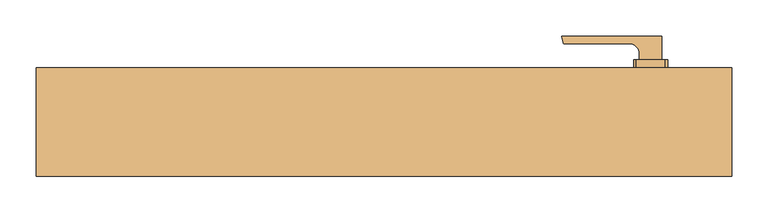
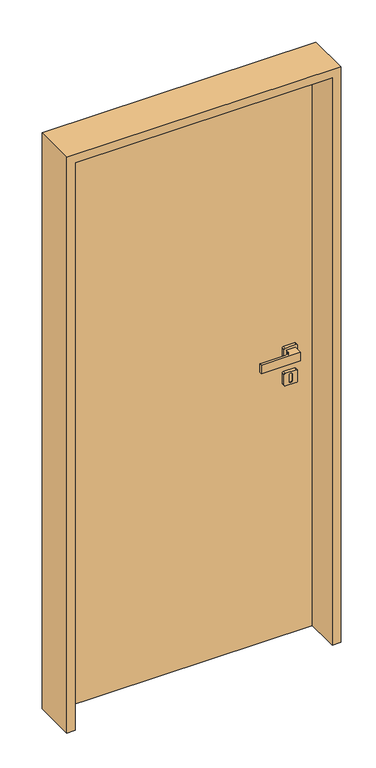
"""IFC4 building model written with IfcOpenShell, lengths in millimetres: door geometry, porta multiplas_growarq : porta giro simples 90 cm_growarq."""

import ifcopenshell
import ifcopenshell.guid

model = None  # the IFC model being written
_history = None  # IfcOwnerHistory: only IFC2X3 demands one
_inside = {}  # id of a spatial element -> (the spatial element, [elements in it])
_under = {}  # id of a project, library or spatial element -> (it, [spatial elements below it])
_declared = {}  # id of a project -> (the project, [libraries it declares])
_typed = {}  # id of a type object -> (the type object, [elements of that type])
_made_of = {}  # id of a material, layer set ... -> (it, [elements and type objects made of it])


def new_model(schema):
    """Start an empty IFC model of exactly this schema.

    Asked for "IFC4X3", IfcOpenShell would pick the latest addendum, in which some entities
    have other attributes; the version numbers below select the first issue.
    IFC2X3 requires an IfcOwnerHistory on every rooted entity: one is made here for all.
    """
    global model, _history
    if schema == "IFC4X3":
        model = ifcopenshell.file(schema_version=(4, 3, 0, 0))
    else:
        model = ifcopenshell.file(schema=schema)
    _inside.clear()
    _under.clear()
    _declared.clear()
    _typed.clear()
    _made_of.clear()
    _history = None
    if model.schema == "IFC2X3":
        org = make("IfcOrganization", Name="unknown")
        user = make(
            "IfcPersonAndOrganization",
            ThePerson=make("IfcPerson", FamilyName="unknown"),
            TheOrganization=org,
        )
        app = make(
            "IfcApplication",
            ApplicationDeveloper=org,
            Version="unknown",
            ApplicationFullName="unknown",
            ApplicationIdentifier="unknown",
        )
        _history = make(
            "IfcOwnerHistory",
            OwningUser=user,
            OwningApplication=app,
            ChangeAction="ADDED",
            CreationDate=0,
        )
    return model


def make(cls, **values):
    """One entity of the class cls with the attributes given. An attribute that is None is left unset."""
    return model.create_entity(
        cls, **{name: value for name, value in values.items() if value is not None}
    )


def rooted(cls, **values):
    """An entity with a GlobalId (a new one), such as an element, a storey or a relation."""
    return make(cls, GlobalId=ifcopenshell.guid.new(), OwnerHistory=_history, **values)


def si_unit(unit_type, name, prefix=None):
    """IfcSIUnit, for example si_unit("LENGTHUNIT", "METRE", prefix="MILLI")."""
    return make("IfcSIUnit", UnitType=unit_type, Prefix=prefix, Name=name)


def assignment(units):
    """IfcUnitAssignment: the units of a project."""
    return None if units is None else make("IfcUnitAssignment", Units=units)


def point(xyz):
    """IfcCartesianPoint."""
    return None if xyz is None else make("IfcCartesianPoint", Coordinates=xyz)


def direction(xyz):
    """IfcDirection."""
    return None if xyz is None else make("IfcDirection", DirectionRatios=xyz)


def frame(location, z_axis=None, x_axis=None):
    """IfcAxis2Placement3D, a coordinate frame: its origin and axes. An axis left out is left unset."""
    return make(
        "IfcAxis2Placement3D",
        Location=point(location),
        Axis=direction(z_axis),
        RefDirection=direction(x_axis),
    )


def frame_2d(location, x_axis=None):
    """IfcAxis2Placement2D, a coordinate frame in the plane: its origin and x axis."""
    return make(
        "IfcAxis2Placement2D", Location=point(location), RefDirection=direction(x_axis)
    )


def origin():
    """The frame at (0, 0, 0) with its axes left unset."""
    return frame((0.0, 0.0, 0.0))


def origin_with_axes():
    """The frame at (0, 0, 0) with the z axis (0, 0, 1) and the x axis (1, 0, 0) written out."""
    return frame((0.0, 0.0, 0.0), z_axis=(0.0, 0.0, 1.0), x_axis=(1.0, 0.0, 0.0))


def place(relative_to, where):
    """IfcLocalPlacement: puts the frame where relative to a parent placement (None: the world)."""
    return make(
        "IfcLocalPlacement", PlacementRelTo=relative_to, RelativePlacement=where
    )


def context(
    kind, dimensions, precision=None, world=None, true_north=None, identifier=None
):
    """IfcGeometricRepresentationContext, for example the 3D "Model" context."""
    return make(
        "IfcGeometricRepresentationContext",
        ContextIdentifier=identifier,
        ContextType=kind,
        CoordinateSpaceDimension=dimensions,
        Precision=precision,
        WorldCoordinateSystem=world,
        TrueNorth=true_north,
    )


def project(units=None, contexts=None):
    """IfcProject with its units and contexts."""
    return rooted(
        "IfcProject",
        Name="project",
        RepresentationContexts=contexts,
        UnitsInContext=assignment(units),
    )


def spatial(cls, under=None, at=None, **own):
    """A site, building, storey or space (cls), placed at a placement, below another one or the project."""
    s = rooted(cls, ObjectPlacement=at, **own)
    if under is not None:
        _under.setdefault(under.id(), (under, []))[1].append(s)
    return s


def polyline(points):
    """IfcPolyline through the points."""
    return make("IfcPolyline", Points=[point(p) for p in points])


def circle_curve(where, radius):
    """IfcCircle in the frame where."""
    return make("IfcCircle", Position=where, Radius=radius)


def trimmed(basis, trim1, trim2, sense, master):
    """IfcTrimmedCurve: the piece of a basis curve between two trims."""
    return make(
        "IfcTrimmedCurve",
        BasisCurve=basis,
        Trim1=trim1,
        Trim2=trim2,
        SenseAgreement=sense,
        MasterRepresentation=master,
    )


def segment(curve, same_sense, transition):
    """IfcCompositeCurveSegment."""
    return make(
        "IfcCompositeCurveSegment",
        Transition=transition,
        SameSense=same_sense,
        ParentCurve=curve,
    )


def composite_curve(segments, self_intersect=None):
    """IfcCompositeCurve: segments joined end to end."""
    return make("IfcCompositeCurve", Segments=segments, SelfIntersect=self_intersect)


def outline(outer, holes=None, kind="AREA"):
    """IfcArbitraryClosedProfileDef: a profile drawn as a closed curve; with holes, ...WithVoids."""
    if holes is None:
        return make("IfcArbitraryClosedProfileDef", ProfileType=kind, OuterCurve=outer)
    return make(
        "IfcArbitraryProfileDefWithVoids",
        ProfileType=kind,
        OuterCurve=outer,
        InnerCurves=holes,
    )


def extrude(swept, where, along, depth):
    """IfcExtrudedAreaSolid: the profile swept, set in the frame where, extruded along a direction by depth."""
    return make(
        "IfcExtrudedAreaSolid",
        SweptArea=swept,
        Position=where,
        ExtrudedDirection=direction(along),
        Depth=depth,
    )


def shape(context_of_items, identifier, shape_type, items):
    """IfcShapeRepresentation: the items that make up one representation, for example the "Body"."""
    return make(
        "IfcShapeRepresentation",
        ContextOfItems=context_of_items,
        RepresentationIdentifier=identifier,
        RepresentationType=shape_type,
        Items=items,
    )


def source(mapping_origin, context_of_items, identifier, shape_type, items):
    """IfcRepresentationMap: a shape defined once, which mapped items show again and again."""
    return make(
        "IfcRepresentationMap",
        MappingOrigin=mapping_origin,
        MappedRepresentation=shape(context_of_items, identifier, shape_type, items),
    )


def transform(
    local_origin,
    x_axis=None,
    y_axis=None,
    z_axis=None,
    scale=None,
    scale2=None,
    scale3=None,
    uniform=True,
):
    """IfcCartesianTransformationOperator3D, or its non-uniform kind. x_axis, y_axis, z_axis: its Axis1, 2, 3."""
    if uniform:
        return make(
            "IfcCartesianTransformationOperator3D",
            Axis1=direction(x_axis),
            Axis2=direction(y_axis),
            LocalOrigin=point(local_origin),
            Scale=scale,
            Axis3=direction(z_axis),
        )
    return make(
        "IfcCartesianTransformationOperator3DnonUniform",
        Axis1=direction(x_axis),
        Axis2=direction(y_axis),
        LocalOrigin=point(local_origin),
        Scale=scale,
        Axis3=direction(z_axis),
        Scale2=scale2,
        Scale3=scale3,
    )


def mapped(mapping_source, mapping_target):
    """IfcMappedItem: shows the shape of a source again, moved by a transform."""
    return make(
        "IfcMappedItem", MappingSource=mapping_source, MappingTarget=mapping_target
    )


def made_of(thing, what):
    """Note that an element or type object is made of a material, layer set ...; save() writes the relation."""
    if what is not None:
        _made_of.setdefault(what.id(), (what, []))[1].append(thing)
    return thing


def element(
    cls,
    number,
    at=None,
    inside=None,
    cuts=None,
    type_object=None,
    material=None,
    context=None,
    identifier="Body",
    shape_type=None,
    held_by="IfcProductDefinitionShape",
    body=None,
    shapes=None,
    **own,
):
    """One element of the class cls, such as IfcWall. Its Tag is "e" and its number.

    at: its placement. inside: the storey or other place that contains it. cuts: it is an
    opening in that element (IfcRelVoidsElement). A single representation is given by context,
    identifier, shape_type and body (its items); several are given by shapes. held_by: the class
    of the entity that holds the representations. save() writes the other relations.
    """
    e = rooted(cls, Tag="e%d" % number, ObjectPlacement=at, **own)
    if body is not None:
        shapes = [shape(context, identifier, shape_type, body)]
    if shapes is not None:
        e.Representation = make(held_by, Representations=shapes)
    if inside is not None:
        _inside.setdefault(inside.id(), (inside, []))[1].append(e)
    if cuts is not None:
        rooted(
            "IfcRelVoidsElement", RelatingBuildingElement=cuts, RelatedOpeningElement=e
        )
    if type_object is not None:
        _typed.setdefault(type_object.id(), (type_object, []))[1].append(e)
    return made_of(e, material)


def aggregate(whole, parts):
    """IfcRelAggregates: a whole, such as a stair, and the parts it consists of."""
    return rooted("IfcRelAggregates", RelatingObject=whole, RelatedObjects=parts)


def save(model, path):
    """Write the relations noted so far, then the file.

    IfcRelAggregates (storeys below a building ...), IfcRelContainedInSpatialStructure (elements
    in a storey), IfcRelDefinesByType, IfcRelAssociatesMaterial and IfcRelDeclares: one each for
    every whole, place, type object, material and project.
    """
    for whole, parts in _under.values():
        aggregate(whole, parts)
    for where, things in _inside.values():
        rooted(
            "IfcRelContainedInSpatialStructure",
            RelatedElements=things,
            RelatingStructure=where,
        )
    for kind, things in _typed.values():
        rooted("IfcRelDefinesByType", RelatedObjects=things, RelatingType=kind)
    for what, things in _made_of.values():
        rooted("IfcRelAssociatesMaterial", RelatedObjects=things, RelatingMaterial=what)
    for by, libraries in _declared.values():
        rooted("IfcRelDeclares", RelatingContext=by, RelatedDefinitions=libraries)
    model.write(path)


def plane_surface(at):
    """IfcPlane: the flat surface through the origin of the frame at, square to its z axis."""
    return make("IfcPlane", Position=at)


def cylinder_surface(at, radius):
    """IfcCylindricalSurface: all points at the distance radius from the z axis of the frame at."""
    return make("IfcCylindricalSurface", Position=at, Radius=radius)


def revolved_surface(curve, axis_point, axis_direction):
    """IfcSurfaceOfRevolution: the curve turned about the line through axis_point along axis_direction."""
    return make(
        "IfcSurfaceOfRevolution",
        SweptCurve=make("IfcArbitraryOpenProfileDef", ProfileType="CURVE", Curve=curve),
        AxisPosition=make("IfcAxis1Placement", Location=point(axis_point), Axis=direction(axis_direction)),
    )


def advanced_brep(points, edges, surfaces, faces):
    """IfcAdvancedBrep: a solid bounded by faces that lie on surfaces and meet in shared edges.

    An edge is (start, end): straight between two places in points (the first is 0);
    or (start, end, curve); or (start, end, curve, False) where it runs against its curve.
    A face is (place in surfaces, loops), or (place, loops, False) where it looks against
    its surface's normal. A loop lists edges by number (the first is 1), with a minus sign
    where the edge is run from its end to its start. The first loop is the outer one.
    """
    corners = [point(p) for p in points]
    vertices = [make("IfcVertexPoint", VertexGeometry=c) for c in corners]
    made = []
    for start, end, *more in edges:
        made.append(
            make(
                "IfcEdgeCurve",
                EdgeStart=vertices[start],
                EdgeEnd=vertices[end],
                EdgeGeometry=more[0] if more else make("IfcPolyline", Points=[corners[start], corners[end]]),
                SameSense=more[1] if len(more) > 1 else True,
            )
        )
    hull = []
    for where, loops, *sense in faces:
        bounds = []
        for j, loop in enumerate(loops):
            ring = [make("IfcOrientedEdge", EdgeElement=made[abs(k) - 1], Orientation=k > 0) for k in loop]
            bounds.append(
                make(
                    "IfcFaceOuterBound" if j == 0 else "IfcFaceBound",
                    Bound=make("IfcEdgeLoop", EdgeList=ring),
                    Orientation=True,
                )
            )
        hull.append(make("IfcAdvancedFace", Bounds=bounds, FaceSurface=surfaces[where], SameSense=sense[0] if sense else True))
    return make("IfcAdvancedBrep", Outer=make("IfcClosedShell", CfsFaces=hull))


def door_3435e1a8(model_context):
    return source(origin(), model_context, "Body", "SolidModel", [
        advanced_brep(
        [(387.5247906, 86.0, 975.2140175), (391.5247906, 86.0, 971.2140175), (391.5247906, 86.0, 932.3348635), (387.5247906, 86.0, 928.3348635), (348.475196, 86.0, 928.3348635), (344.475196, 86.0, 932.3348635), (344.475196, 86.0, 971.2071442), (348.4820692, 86.0, 975.2140175), (373.0036235, 86.0, 963.1453546), (362.9935514, 86.0, 963.1453546), (362.9935514, 86.0, 940.4035264), (373.0036235, 86.0, 940.4035264), (387.5247906, 75.0, 975.2140175), (348.4820692, 75.0, 975.2140175), (344.475196, 75.0, 971.2071442), (344.475196, 75.0, 932.3348635), (348.475196, 75.0, 928.3348635), (387.5247906, 75.0, 928.3348635), (391.5247906, 75.0, 932.3348635), (391.5247906, 75.0, 971.2140175), (373.0036235, 84.0, 940.4035264), (362.9935514, 84.0, 940.4035264), (362.9935514, 84.0, 963.1453546), (373.0036235, 84.0, 963.1453546)],
        [
            (0, 1, circle_curve(frame((387.5247906, 86.0, 971.2140175), z_axis=(0.0, 1.0, 0.0), x_axis=(1.0, 0.0, 0.0)), 4.0)),
            (1, 2),
            (2, 3, circle_curve(frame((387.5247906, 86.0, 932.3348635), z_axis=(0.0, 1.0, 0.0), x_axis=(1.0, 0.0, 0.0)), 4.0)),
            (3, 4),
            (4, 5, circle_curve(frame((348.475196, 86.0, 932.3348635), z_axis=(0.0, 1.0, 0.0), x_axis=(1.0, 0.0, 0.0)), 4.0)),
            (5, 6),
            (6, 7, circle_curve(frame((348.4820692, 86.0, 971.2071442), z_axis=(0.0, 1.0, 0.0), x_axis=(1.0, 0.0, 0.0)), 4.0068732)),
            (7, 0),
            (8, 9, circle_curve(frame((367.9985874, 86.0, 963.1453546), z_axis=(0.0, -1.0, 0.0), x_axis=(1.0, 0.0, 0.0)), 5.0050361)),
            (9, 10),
            (10, 11, circle_curve(frame((367.9985874, 86.0, 940.4035264), z_axis=(0.0, -1.0, 0.0), x_axis=(1.0, 0.0, 0.0)), 5.0050361)),
            (11, 8),
            (12, 13),
            (13, 14, circle_curve(frame((348.4820692, 75.0, 971.2071442), z_axis=(0.0, -1.0, 0.0), x_axis=(1.0, 0.0, 0.0)), 4.0068732)),
            (14, 15),
            (15, 16, circle_curve(frame((348.475196, 75.0, 932.3348635), z_axis=(0.0, -1.0, 0.0), x_axis=(1.0, 0.0, 0.0)), 4.0)),
            (16, 17),
            (17, 18, circle_curve(frame((387.5247906, 75.0, 932.3348635), z_axis=(0.0, -1.0, 0.0), x_axis=(1.0, 0.0, 0.0)), 4.0)),
            (18, 19),
            (19, 12, circle_curve(frame((387.5247906, 75.0, 971.2140175), z_axis=(0.0, -1.0, 0.0), x_axis=(1.0, 0.0, 0.0)), 4.0)),
            (7, 13),
            (12, 0),
            (6, 14),
            (5, 15),
            (4, 16),
            (3, 17),
            (2, 18),
            (1, 19),
            (20, 21, circle_curve(frame((367.9985874, 84.0, 940.4035264), z_axis=(0.0, 1.0, 0.0), x_axis=(1.0, 0.0, 0.0)), 5.0050361)),
            (21, 22),
            (22, 23, circle_curve(frame((367.9985874, 84.0, 963.1453546), z_axis=(0.0, 1.0, 0.0), x_axis=(1.0, 0.0, 0.0)), 5.0050361)),
            (23, 20),
            (23, 8),
            (11, 20),
            (21, 10),
            (9, 22),
        ],
        [
            plane_surface(frame((348.4781039, 86.0, 975.2140175), z_axis=(0.0, 1.0, 0.0), x_axis=(-1.0, 0.0, 0.0))),
            plane_surface(frame((348.4781039, 75.0, 975.2140175), z_axis=(0.0, -1.0, 0.0), x_axis=(1.0, 0.0, 0.0))),
            plane_surface(frame((387.5247906, 86.0, 975.2140175), z_axis=(0.0, 0.0, 1.0), x_axis=(0.0, -1.0, 0.0))),
            cylinder_surface(frame((348.4820692, 75.0, 971.2071442), z_axis=(0.0, 1.0, 0.0), x_axis=(1.0, 0.0, 0.0)), 4.0068732),
            plane_surface(frame((344.475196, 86.0, 971.2071442), z_axis=(-1.0, 0.0, 0.0), x_axis=(0.0, -1.0, 0.0))),
            cylinder_surface(frame((348.475196, 75.0, 932.3348635), z_axis=(0.0, 1.0, 0.0), x_axis=(1.0, 0.0, 0.0)), 4.0),
            plane_surface(frame((348.475196, 86.0, 928.3348635), z_axis=(0.0, 0.0, -1.0), x_axis=(0.0, -1.0, 0.0))),
            cylinder_surface(frame((387.5247906, 75.0, 932.3348635), z_axis=(0.0, 1.0, 0.0), x_axis=(1.0, 0.0, 0.0)), 4.0),
            plane_surface(frame((391.5247906, 86.0, 932.3348635), z_axis=(1.0, 0.0, 0.0), x_axis=(0.0, -1.0, 0.0))),
            cylinder_surface(frame((387.5247906, 75.0, 971.2140175), z_axis=(0.0, 1.0, 0.0), x_axis=(1.0, 0.0, 0.0)), 4.0),
            plane_surface(frame((373.0036235, 84.0, 952.9958878), z_axis=(0.0, 1.0, 0.0), x_axis=(0.0, 0.0, -1.0))),
            plane_surface(frame((373.0036235, 86.0, 940.4035264), z_axis=(-1.0, 0.0, 0.0), x_axis=(0.0, -1.0, 0.0))),
            plane_surface(frame((362.9935514, 86.0, 963.1453546), z_axis=(1.0, 0.0, 0.0), x_axis=(0.0, -1.0, 0.0))),
            revolved_surface(polyline([(373.0036235, 86.0, 940.4035264), (373.0036235, 84.0, 940.4035264)]), (367.9985874, 84.0, 940.4035264), (0.0, 1.0, 0.0)),
            revolved_surface(polyline([(373.0036235, 86.0, 963.1453546), (373.0036235, 84.0, 963.1453546)]), (367.9985874, 84.0, 963.1453546), (0.0, 1.0, 0.0)),
        ],
        [
            (0, [[1, 2, 3, 4, 5, 6, 7, 8], [9, 10, 11, 12]]),
            (1, [[13, 14, 15, 16, 17, 18, 19, 20]]),
            (2, [[21, -13, 22, -8]]),
            (3, [[23, -14, -21, -7]]),
            (4, [[24, -15, -23, -6]]),
            (5, [[25, -16, -24, -5]]),
            (6, [[26, -17, -25, -4]]),
            (7, [[27, -18, -26, -3]]),
            (8, [[28, -19, -27, -2]]),
            (9, [[-22, -20, -28, -1]]),
            (10, [[29, 30, 31, 32]]),
            (11, [[33, -12, 34, -32]]),
            (12, [[35, -10, 36, -30]]),
            (13, [[-34, -11, -35, -29]]),
            (14, [[-36, -9, -33, -31]]),
        ],
    ),
        advanced_brep(
        [(387.5247906, 86.0, 1068.227973), (391.5247906, 86.0, 1064.227973), (391.5247906, 86.0, 1025.3488191), (387.5247906, 86.0, 1021.3488191), (348.475196, 86.0, 1021.3488191), (344.475196, 86.0, 1025.3488191), (344.475196, 86.0, 1064.2210998), (348.4820692, 86.0, 1068.227973), (387.5247906, 75.0, 1068.227973), (348.4820692, 75.0, 1068.227973), (344.475196, 75.0, 1064.2210998), (344.475196, 75.0, 1025.3488191), (348.475196, 75.0, 1021.3488191), (387.5247906, 75.0, 1021.3488191), (391.5247906, 75.0, 1025.3488191), (391.5247906, 75.0, 1064.227973)],
        [
            (0, 1, circle_curve(frame((387.5247906, 86.0, 1064.227973), z_axis=(0.0, 1.0, 0.0), x_axis=(1.0, 0.0, 0.0)), 4.0)),
            (1, 2),
            (2, 3, circle_curve(frame((387.5247906, 86.0, 1025.3488191), z_axis=(0.0, 1.0, 0.0), x_axis=(1.0, 0.0, 0.0)), 4.0)),
            (3, 4),
            (4, 5, circle_curve(frame((348.475196, 86.0, 1025.3488191), z_axis=(0.0, 1.0, 0.0), x_axis=(1.0, 0.0, 0.0)), 4.0)),
            (5, 6),
            (6, 7, circle_curve(frame((348.4820692, 86.0, 1064.2210998), z_axis=(0.0, 1.0, 0.0), x_axis=(1.0, 0.0, 0.0)), 4.0068732)),
            (7, 0),
            (8, 9),
            (9, 10, circle_curve(frame((348.4820692, 75.0, 1064.2210998), z_axis=(0.0, -1.0, 0.0), x_axis=(1.0, 0.0, 0.0)), 4.0068732)),
            (10, 11),
            (11, 12, circle_curve(frame((348.475196, 75.0, 1025.3488191), z_axis=(0.0, -1.0, 0.0), x_axis=(1.0, 0.0, 0.0)), 4.0)),
            (12, 13),
            (13, 14, circle_curve(frame((387.5247906, 75.0, 1025.3488191), z_axis=(0.0, -1.0, 0.0), x_axis=(1.0, 0.0, 0.0)), 4.0)),
            (14, 15),
            (15, 8, circle_curve(frame((387.5247906, 75.0, 1064.227973), z_axis=(0.0, -1.0, 0.0), x_axis=(1.0, 0.0, 0.0)), 4.0)),
            (7, 9),
            (8, 0),
            (6, 10),
            (5, 11),
            (4, 12),
            (3, 13),
            (2, 14),
            (1, 15),
        ],
        [
            plane_surface(frame((348.4781039, 86.0, 975.2140175), z_axis=(0.0, 1.0, 0.0), x_axis=(-1.0, 0.0, 0.0))),
            plane_surface(frame((348.4781039, 75.0, 975.2140175), z_axis=(0.0, -1.0, 0.0), x_axis=(1.0, 0.0, 0.0))),
            plane_surface(frame((387.5247906, 86.0, 1068.227973), z_axis=(0.0, 0.0, 1.0), x_axis=(0.0, -1.0, 0.0))),
            cylinder_surface(frame((348.4820692, 75.0, 1064.2210998), z_axis=(0.0, 1.0, 0.0), x_axis=(1.0, 0.0, 0.0)), 4.0068732),
            plane_surface(frame((344.475196, 86.0, 1064.2210998), z_axis=(-1.0, 0.0, 0.0), x_axis=(0.0, -1.0, 0.0))),
            cylinder_surface(frame((348.475196, 75.0, 1025.3488191), z_axis=(0.0, 1.0, 0.0), x_axis=(1.0, 0.0, 0.0)), 4.0),
            plane_surface(frame((348.475196, 86.0, 1021.3488191), z_axis=(0.0, 0.0, -1.0), x_axis=(0.0, -1.0, 0.0))),
            cylinder_surface(frame((387.5247906, 75.0, 1025.3488191), z_axis=(0.0, 1.0, 0.0), x_axis=(1.0, 0.0, 0.0)), 4.0),
            plane_surface(frame((391.5247906, 86.0, 1025.3488191), z_axis=(1.0, 0.0, 0.0), x_axis=(0.0, -1.0, 0.0))),
            cylinder_surface(frame((387.5247906, 75.0, 1064.227973), z_axis=(0.0, 1.0, 0.0), x_axis=(1.0, 0.0, 0.0)), 4.0),
        ],
        [
            (0, [[1, 2, 3, 4, 5, 6, 7, 8]]),
            (1, [[9, 10, 11, 12, 13, 14, 15, 16]]),
            (2, [[17, -9, 18, -8]]),
            (3, [[19, -10, -17, -7]]),
            (4, [[20, -11, -19, -6]]),
            (5, [[21, -12, -20, -5]]),
            (6, [[22, -13, -21, -4]]),
            (7, [[23, -14, -22, -3]]),
            (8, [[24, -15, -23, -2]]),
            (9, [[-18, -16, -24, -1]]),
        ],
    ),
        extrude(outline(composite_curve([segment(polyline([(383.5247906, 118.5150355), (383.5247906, 86.7793682), (352.475196, 86.7793682), (352.475196, 93.5981558)]), True, "CONTINUOUS"), segment(trimmed(circle_curve(frame_2d((337.4483579, 93.5981558)), 15.0268381), [point((352.475196, 93.5981558))], [point((337.4483579, 108.6249939))], True, "CARTESIAN"), True, "CONTINUOUS"), segment(polyline([(337.4483579, 108.6249939), (248.1590205, 108.6249939)]), True, "CONTINUOUS"), segment(trimmed(circle_curve(frame_2d((248.1590205, 109.6372538)), 1.0122598), [point((248.1590205, 108.6249939))], [point((247.1621392, 109.4614767))], False, "CARTESIAN"), True, "CONTINUOUS"), segment(polyline([(247.1621392, 109.4614767), (245.5657525, 118.5150355), (383.5247906, 118.5150355)]), True, "CONTINUOUS")], self_intersect=False)), frame((0.0, 0.0, 1029.3488191), z_axis=(0.0, 0.0, 1.0), x_axis=(1.0, 0.0, 0.0)), (0.0, 0.0, 1.0), 30.8791539),
        advanced_brep(
        [(387.5247906, 34.0, 975.2140175), (348.4820692, 34.0, 975.2140175), (344.475196, 34.0, 971.2071442), (344.475196, 34.0, 932.3348635), (348.475196, 34.0, 928.3348635), (387.5247906, 34.0, 928.3348635), (391.5247906, 34.0, 932.3348635), (391.5247906, 34.0, 971.2140175), (373.0036235, 34.0, 963.1453546), (373.0036235, 34.0, 940.4035264), (362.9935514, 34.0, 940.4035264), (362.9935514, 34.0, 963.1453546), (387.5247906, 45.0, 975.2140175), (391.5247906, 45.0, 971.2140175), (391.5247906, 45.0, 932.3348635), (387.5247906, 45.0, 928.3348635), (348.475196, 45.0, 928.3348635), (344.475196, 45.0, 932.3348635), (344.475196, 45.0, 971.2071442), (348.4820692, 45.0, 975.2140175), (373.0036235, 36.0, 940.4035264), (373.0036235, 36.0, 963.1453546), (362.9935514, 36.0, 963.1453546), (362.9935514, 36.0, 940.4035264)],
        [
            (0, 1),
            (1, 2, circle_curve(frame((348.4820692, 34.0, 971.2071442), z_axis=(0.0, -1.0, 0.0), x_axis=(1.0, 0.0, 0.0)), 4.0068732)),
            (2, 3),
            (3, 4, circle_curve(frame((348.475196, 34.0, 932.3348635), z_axis=(0.0, -1.0, 0.0), x_axis=(1.0, 0.0, 0.0)), 4.0)),
            (4, 5),
            (5, 6, circle_curve(frame((387.5247906, 34.0, 932.3348635), z_axis=(0.0, -1.0, 0.0), x_axis=(1.0, 0.0, 0.0)), 4.0)),
            (6, 7),
            (7, 0, circle_curve(frame((387.5247906, 34.0, 971.2140175), z_axis=(0.0, -1.0, 0.0), x_axis=(1.0, 0.0, 0.0)), 4.0)),
            (8, 9),
            (9, 10, circle_curve(frame((367.9985874, 34.0, 940.4035264), z_axis=(0.0, 1.0, 0.0), x_axis=(1.0, 0.0, 0.0)), 5.0050361)),
            (10, 11),
            (11, 8, circle_curve(frame((367.9985874, 34.0, 963.1453546), z_axis=(0.0, 1.0, 0.0), x_axis=(1.0, 0.0, 0.0)), 5.0050361)),
            (12, 13, circle_curve(frame((387.5247906, 45.0, 971.2140175), z_axis=(0.0, 1.0, 0.0), x_axis=(1.0, 0.0, 0.0)), 4.0)),
            (13, 14),
            (14, 15, circle_curve(frame((387.5247906, 45.0, 932.3348635), z_axis=(0.0, 1.0, 0.0), x_axis=(1.0, 0.0, 0.0)), 4.0)),
            (15, 16),
            (16, 17, circle_curve(frame((348.475196, 45.0, 932.3348635), z_axis=(0.0, 1.0, 0.0), x_axis=(1.0, 0.0, 0.0)), 4.0)),
            (17, 18),
            (18, 19, circle_curve(frame((348.4820692, 45.0, 971.2071442), z_axis=(0.0, 1.0, 0.0), x_axis=(1.0, 0.0, 0.0)), 4.0068732)),
            (19, 12),
            (0, 12),
            (19, 1),
            (18, 2),
            (17, 3),
            (16, 4),
            (15, 5),
            (14, 6),
            (13, 7),
            (20, 21),
            (21, 22, circle_curve(frame((367.9985874, 36.0, 963.1453546), z_axis=(0.0, -1.0, 0.0), x_axis=(1.0, 0.0, 0.0)), 5.0050361)),
            (22, 23),
            (23, 20, circle_curve(frame((367.9985874, 36.0, 940.4035264), z_axis=(0.0, -1.0, 0.0), x_axis=(1.0, 0.0, 0.0)), 5.0050361)),
            (20, 9),
            (8, 21),
            (22, 11),
            (10, 23),
        ],
        [
            plane_surface(frame((348.4781039, 34.0, 975.2140175), z_axis=(0.0, -1.0, 0.0), x_axis=(-1.0, 0.0, 0.0))),
            plane_surface(frame((348.4781039, 45.0, 975.2140175), z_axis=(0.0, 1.0, 0.0), x_axis=(1.0, 0.0, 0.0))),
            plane_surface(frame((387.5247906, 34.0, 975.2140175), z_axis=(0.0, 0.0, 1.0), x_axis=(0.0, 1.0, 0.0))),
            cylinder_surface(frame((348.4820692, 45.0, 971.2071442), z_axis=(0.0, -1.0, 0.0), x_axis=(1.0, 0.0, 0.0)), 4.0068732),
            plane_surface(frame((344.475196, 34.0, 971.2071442), z_axis=(-1.0, 0.0, 0.0), x_axis=(0.0, 1.0, 0.0))),
            cylinder_surface(frame((348.475196, 45.0, 932.3348635), z_axis=(0.0, -1.0, 0.0), x_axis=(1.0, 0.0, 0.0)), 4.0),
            plane_surface(frame((348.475196, 34.0, 928.3348635), z_axis=(0.0, 0.0, -1.0), x_axis=(0.0, 1.0, 0.0))),
            cylinder_surface(frame((387.5247906, 45.0, 932.3348635), z_axis=(0.0, -1.0, 0.0), x_axis=(1.0, 0.0, 0.0)), 4.0),
            plane_surface(frame((391.5247906, 34.0, 932.3348635), z_axis=(1.0, 0.0, 0.0), x_axis=(0.0, 1.0, 0.0))),
            cylinder_surface(frame((387.5247906, 45.0, 971.2140175), z_axis=(0.0, -1.0, 0.0), x_axis=(1.0, 0.0, 0.0)), 4.0),
            plane_surface(frame((373.0036235, 36.0, 952.9958878), z_axis=(0.0, -1.0, 0.0), x_axis=(0.0, 0.0, -1.0))),
            plane_surface(frame((373.0036235, 34.0, 940.4035264), z_axis=(-1.0, 0.0, 0.0), x_axis=(0.0, 1.0, 0.0))),
            plane_surface(frame((362.9935514, 34.0, 963.1453546), z_axis=(1.0, 0.0, 0.0), x_axis=(0.0, 1.0, 0.0))),
            revolved_surface(polyline([(373.0036235, 34.0, 940.4035264), (373.0036235, 36.0, 940.4035264)]), (367.9985874, 36.0, 940.4035264), (0.0, -1.0, 0.0)),
            revolved_surface(polyline([(373.0036235, 34.0, 963.1453546), (373.0036235, 36.0, 963.1453546)]), (367.9985874, 36.0, 963.1453546), (0.0, -1.0, 0.0)),
        ],
        [
            (0, [[1, 2, 3, 4, 5, 6, 7, 8], [9, 10, 11, 12]]),
            (1, [[13, 14, 15, 16, 17, 18, 19, 20]]),
            (2, [[-1, 21, -20, 22]]),
            (3, [[-2, -22, -19, 23]]),
            (4, [[-3, -23, -18, 24]]),
            (5, [[-4, -24, -17, 25]]),
            (6, [[-5, -25, -16, 26]]),
            (7, [[-6, -26, -15, 27]]),
            (8, [[-7, -27, -14, 28]]),
            (9, [[-8, -28, -13, -21]]),
            (10, [[29, 30, 31, 32]]),
            (11, [[-29, 33, -9, 34]]),
            (12, [[-31, 35, -11, 36]]),
            (13, [[-32, -36, -10, -33]]),
            (14, [[-30, -34, -12, -35]]),
        ],
    ),
        advanced_brep(
        [(387.5247906, 34.0, 1068.227973), (348.4820692, 34.0, 1068.227973), (344.475196, 34.0, 1064.2210998), (344.475196, 34.0, 1025.3488191), (348.475196, 34.0, 1021.3488191), (387.5247906, 34.0, 1021.3488191), (391.5247906, 34.0, 1025.3488191), (391.5247906, 34.0, 1064.227973), (387.5247906, 45.0, 1068.227973), (391.5247906, 45.0, 1064.227973), (391.5247906, 45.0, 1025.3488191), (387.5247906, 45.0, 1021.3488191), (348.475196, 45.0, 1021.3488191), (344.475196, 45.0, 1025.3488191), (344.475196, 45.0, 1064.2210998), (348.4820692, 45.0, 1068.227973)],
        [
            (0, 1),
            (1, 2, circle_curve(frame((348.4820692, 34.0, 1064.2210998), z_axis=(0.0, -1.0, 0.0), x_axis=(1.0, 0.0, 0.0)), 4.0068732)),
            (2, 3),
            (3, 4, circle_curve(frame((348.475196, 34.0, 1025.3488191), z_axis=(0.0, -1.0, 0.0), x_axis=(1.0, 0.0, 0.0)), 4.0)),
            (4, 5),
            (5, 6, circle_curve(frame((387.5247906, 34.0, 1025.3488191), z_axis=(0.0, -1.0, 0.0), x_axis=(1.0, 0.0, 0.0)), 4.0)),
            (6, 7),
            (7, 0, circle_curve(frame((387.5247906, 34.0, 1064.227973), z_axis=(0.0, -1.0, 0.0), x_axis=(1.0, 0.0, 0.0)), 4.0)),
            (8, 9, circle_curve(frame((387.5247906, 45.0, 1064.227973), z_axis=(0.0, 1.0, 0.0), x_axis=(1.0, 0.0, 0.0)), 4.0)),
            (9, 10),
            (10, 11, circle_curve(frame((387.5247906, 45.0, 1025.3488191), z_axis=(0.0, 1.0, 0.0), x_axis=(1.0, 0.0, 0.0)), 4.0)),
            (11, 12),
            (12, 13, circle_curve(frame((348.475196, 45.0, 1025.3488191), z_axis=(0.0, 1.0, 0.0), x_axis=(1.0, 0.0, 0.0)), 4.0)),
            (13, 14),
            (14, 15, circle_curve(frame((348.4820692, 45.0, 1064.2210998), z_axis=(0.0, 1.0, 0.0), x_axis=(1.0, 0.0, 0.0)), 4.0068732)),
            (15, 8),
            (0, 8),
            (15, 1),
            (14, 2),
            (13, 3),
            (12, 4),
            (11, 5),
            (10, 6),
            (9, 7),
        ],
        [
            plane_surface(frame((348.4781039, 34.0, 975.2140175), z_axis=(0.0, -1.0, 0.0), x_axis=(-1.0, 0.0, 0.0))),
            plane_surface(frame((348.4781039, 45.0, 975.2140175), z_axis=(0.0, 1.0, 0.0), x_axis=(1.0, 0.0, 0.0))),
            plane_surface(frame((387.5247906, 34.0, 1068.227973), z_axis=(0.0, 0.0, 1.0), x_axis=(0.0, 1.0, 0.0))),
            cylinder_surface(frame((348.4820692, 45.0, 1064.2210998), z_axis=(0.0, -1.0, 0.0), x_axis=(1.0, 0.0, 0.0)), 4.0068732),
            plane_surface(frame((344.475196, 34.0, 1064.2210998), z_axis=(-1.0, 0.0, 0.0), x_axis=(0.0, 1.0, 0.0))),
            cylinder_surface(frame((348.475196, 45.0, 1025.3488191), z_axis=(0.0, -1.0, 0.0), x_axis=(1.0, 0.0, 0.0)), 4.0),
            plane_surface(frame((348.475196, 34.0, 1021.3488191), z_axis=(0.0, 0.0, -1.0), x_axis=(0.0, 1.0, 0.0))),
            cylinder_surface(frame((387.5247906, 45.0, 1025.3488191), z_axis=(0.0, -1.0, 0.0), x_axis=(1.0, 0.0, 0.0)), 4.0),
            plane_surface(frame((391.5247906, 34.0, 1025.3488191), z_axis=(1.0, 0.0, 0.0), x_axis=(0.0, 1.0, 0.0))),
            cylinder_surface(frame((387.5247906, 45.0, 1064.227973), z_axis=(0.0, -1.0, 0.0), x_axis=(1.0, 0.0, 0.0)), 4.0),
        ],
        [
            (0, [[1, 2, 3, 4, 5, 6, 7, 8]]),
            (1, [[9, 10, 11, 12, 13, 14, 15, 16]]),
            (2, [[-1, 17, -16, 18]]),
            (3, [[-2, -18, -15, 19]]),
            (4, [[-3, -19, -14, 20]]),
            (5, [[-4, -20, -13, 21]]),
            (6, [[-5, -21, -12, 22]]),
            (7, [[-6, -22, -11, 23]]),
            (8, [[-7, -23, -10, 24]]),
            (9, [[-8, -24, -9, -17]]),
        ],
    ),
        extrude(outline(composite_curve([segment(polyline([(383.5247906, 1.4849645), (245.5657525, 1.4849645), (247.1621392, 10.5385233)]), True, "CONTINUOUS"), segment(trimmed(circle_curve(frame_2d((248.1590205, 10.3627462)), 1.0122598), [point((247.1621392, 10.5385233))], [point((248.1590205, 11.3750061))], False, "CARTESIAN"), True, "CONTINUOUS"), segment(polyline([(248.1590205, 11.3750061), (337.4483579, 11.3750061)]), True, "CONTINUOUS"), segment(trimmed(circle_curve(frame_2d((337.4483579, 26.4018442)), 15.0268381), [point((337.4483579, 11.3750061))], [point((352.475196, 26.4018442))], True, "CARTESIAN"), True, "CONTINUOUS"), segment(polyline([(352.475196, 26.4018442), (352.475196, 33.2206318), (383.5247906, 33.2206318), (383.5247906, 1.4849645)]), True, "CONTINUOUS")], self_intersect=False)), frame((0.0, 0.0, 1029.3488191), z_axis=(0.0, 0.0, 1.0), x_axis=(1.0, 0.0, 0.0)), (0.0, 0.0, 1.0), 30.8791539),
        extrude(outline(polyline([(448.0, 45.0), (-448.0, 45.0), (-448.0, 75.0), (448.0, 75.0), (448.0, 45.0)])), origin_with_axes(), (0.0, 0.0, 1.0), 2098.0),
        extrude(outline(polyline([(0.0, 450.0), (0.0, 480.0), (2130.0, 480.0), (2130.0, -480.0), (0.0, -480.0), (0.0, -450.0), (2100.0, -450.0), (2100.0, 450.0), (0.0, 450.0)])), frame((0.0, -75.0, 0.0), z_axis=(0.0, 1.0, 0.0), x_axis=(0.0, 0.0, 1.0)), (0.0, 0.0, 1.0), 150.0),
    ])


if __name__ == "__main__":
    model = new_model("IFC4")
    model_context = context("Model", 3, world=origin())
    ifc_project = project(units=[si_unit("LENGTHUNIT", "METRE", prefix="MILLI")], contexts=[model_context])
    site = spatial("IfcSite", under=ifc_project)
    building = spatial("IfcBuilding", under=site)
    placement = place(None, origin())
    door_shape = door_3435e1a8(model_context)
    element("IfcDoor", 1, ObjectType="porta multiplas_growarq : porta giro simples 90 cm_growarq", at=placement, inside=building, context=model_context, shape_type="MappedRepresentation", body=[
        mapped(door_shape, transform((0.0, 0.0, 0.0), x_axis=(1.0, 0.0, 0.0), y_axis=(0.0, 1.0, 0.0), z_axis=(0.0, 0.0, 1.0))),
    ])
    save(model, "model.ifc")

# Revit data of these elements
# Type "porta multiplas_growarq : porta giro simples 90 cm_growarq"
#   Type Mark = "P01"
#   Description = "Porta de Madeira com uma folha de abrir"
#   Analytic Construction = "<None>"
#   Cost = 0
#   Rough Width = 960 mm
#   Largura Guarnição = 50 mm
#   Espessura Guarnição = 10 mm
#   Thickness = 30 mm
#   Rough Height = 2130 mm
#   Marco = 30 mm
#   Largura Folha Eixo = 696 mm
#   Height = 2100 mm
#   Width = 900 mm
#   Largura Folha = 896 mm
#   Eixo = 200 mm
#   Altura Folha = 2098 mm
#   Abertura correr [instance default] = 200 mm
#   Abertura [instance default] = 0.00°
#   Simples = yes
#   Guarnição = no
#   Eixo Folha = no
#   Dupla = no
#   Correr = no
#   Material = .pintura branca_growarq
#   Function = (empty or 0)
#   Wall Closure = (empty or 0)
# Element 1 (IfcDoor, "porta multiplas_growarq : porta giro simples 90 cm_growarq")
#   Materials on its faces: ".pintura branca_growarq"
# Materials
#   ".pintura branca_growarq": class "Pintura", colour RGB 255 255 255, transparency 0, Keynote = "0102", Comments = "Pintura com tinta látex na cor branca", Description = "Pintura branca", Cost = 0
